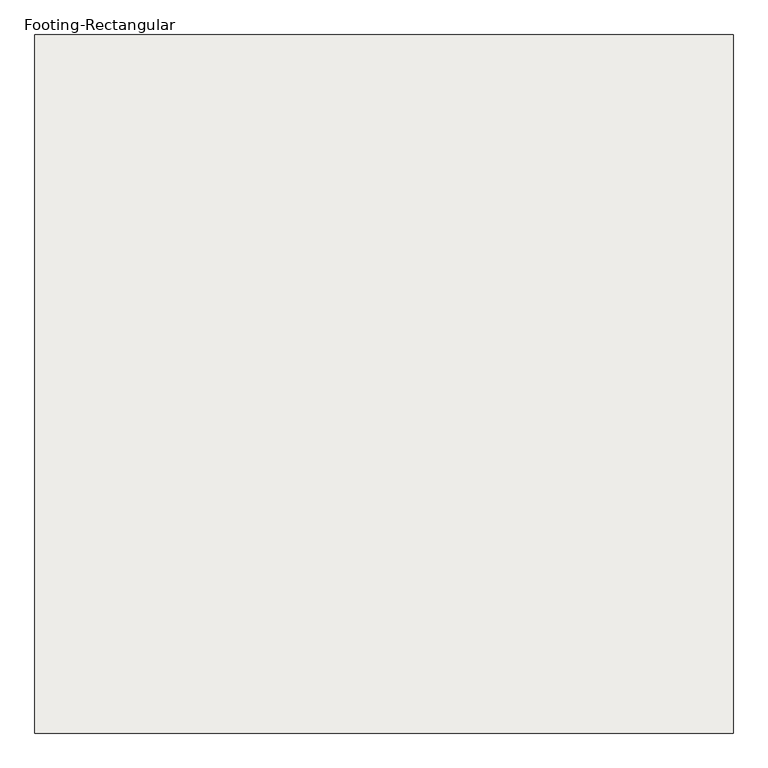
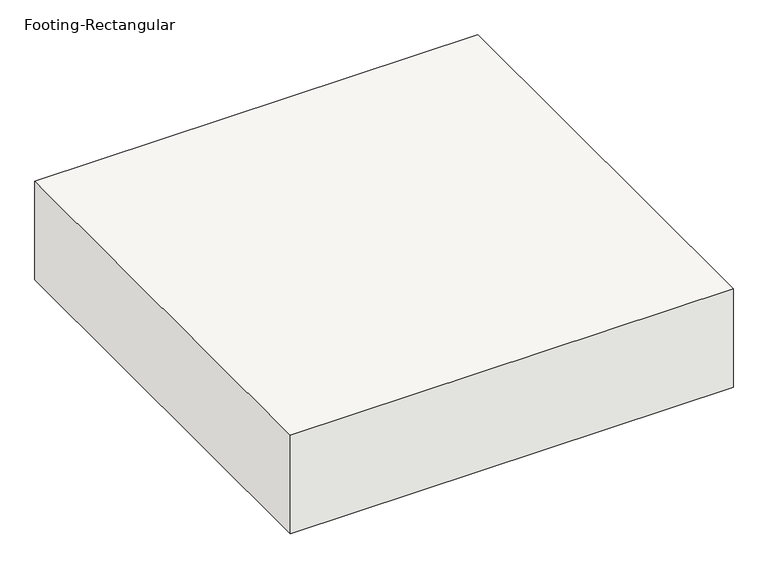
"""IFC4 building model written with IfcOpenShell, lengths in millimetres: slab geometry, Footing-Rectangular."""

from ifc_helpers import new_model, si_unit, frame, origin, place, context, project, spatial, polyline, outline, extrude, source, transform, mapped, element, save


def footing_rectangular_4c268a4d(model_context):
    return source(origin(), model_context, "Body", "SweptSolid", [
        extrude(outline(polyline([(1295.4, 1295.4), (1295.4, -1295.4), (-1295.4, -1295.4), (-1295.4, 1295.4), (1295.4, 1295.4)])), frame((0.0, 0.0, -609.6), z_axis=(0.0, 0.0, 1.0), x_axis=(1.0, 0.0, 0.0)), (0.0, 0.0, 1.0), 609.6),
    ])


if __name__ == "__main__":
    model = new_model("IFC4")
    model_context = context("Model", 3, world=origin())
    ifc_project = project(units=[si_unit("LENGTHUNIT", "METRE", prefix="MILLI")], contexts=[model_context])
    site = spatial("IfcSite", under=ifc_project)
    building = spatial("IfcBuilding", under=site)
    placement = place(None, origin())
    footing_rectangular_shape = footing_rectangular_4c268a4d(model_context)
    element("IfcSlab", 1, ObjectType="Footing-Rectangular : F 8.5' x 8.5' x 24\"", at=placement, inside=building, context=model_context, shape_type="MappedRepresentation", body=[
        mapped(footing_rectangular_shape, transform((0.0, 0.0, 0.0), x_axis=(1.0, 0.0, 0.0), y_axis=(0.0, 1.0, 0.0), z_axis=(0.0, 0.0, 1.0))),
    ])
    save(model, "model.ifc")

# Revit data of these elements
# Type "Footing-Rectangular : F 8.5' x 8.5' x 24\""
#   Assembly Code = "A1010100"
#   Width = 8' - 6"
#   Length = 8' - 6"
#   Foundation Thickness = 2' - 0"
#   Structural Material [instance default] = Concrete, Cast-in-Place gray
# Element 1 (IfcSlab, "Footing-Rectangular : F 8.5' x 8.5' x 24\"")
#   Materials on its faces: "Concrete, Cast-in-Place gray"
# Materials
#   "Concrete, Cast-in-Place gray": class "Concrete", colour RGB 192 192 192, transparency 0, Description = "Cast-in-place concrete", Cost = 0
